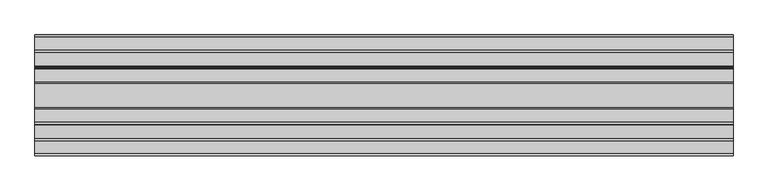
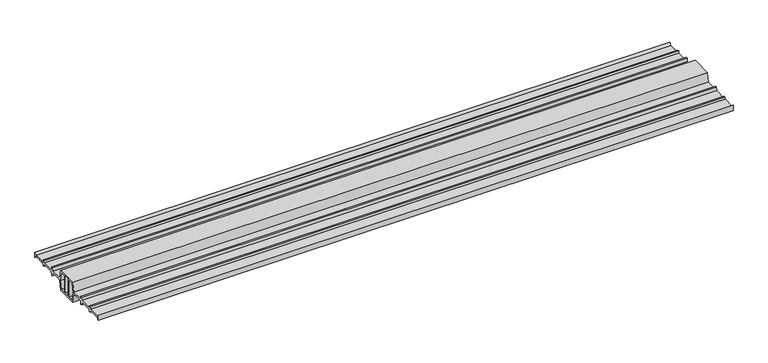
"""IFC4 building model written with IfcOpenShell, lengths in millimetres: proxy geometry, TN_ПВХ_ТПО_Гидрошпонка ТехноНИКОЛЬ : ПВХ Гидрошпонка ТехноНИКОЛЬ IM-260/50."""

import ifcopenshell
import ifcopenshell.guid

model = None  # the IFC model being written
_history = None  # IfcOwnerHistory: only IFC2X3 demands one
_inside = {}  # id of a spatial element -> (the spatial element, [elements in it])
_under = {}  # id of a project, library or spatial element -> (it, [spatial elements below it])
_declared = {}  # id of a project -> (the project, [libraries it declares])
_typed = {}  # id of a type object -> (the type object, [elements of that type])
_made_of = {}  # id of a material, layer set ... -> (it, [elements and type objects made of it])


def new_model(schema):
    """Start an empty IFC model of exactly this schema.

    Asked for "IFC4X3", IfcOpenShell would pick the latest addendum, in which some entities
    have other attributes; the version numbers below select the first issue.
    IFC2X3 requires an IfcOwnerHistory on every rooted entity: one is made here for all.
    """
    global model, _history
    if schema == "IFC4X3":
        model = ifcopenshell.file(schema_version=(4, 3, 0, 0))
    else:
        model = ifcopenshell.file(schema=schema)
    _inside.clear()
    _under.clear()
    _declared.clear()
    _typed.clear()
    _made_of.clear()
    _history = None
    if model.schema == "IFC2X3":
        org = make("IfcOrganization", Name="unknown")
        user = make(
            "IfcPersonAndOrganization",
            ThePerson=make("IfcPerson", FamilyName="unknown"),
            TheOrganization=org,
        )
        app = make(
            "IfcApplication",
            ApplicationDeveloper=org,
            Version="unknown",
            ApplicationFullName="unknown",
            ApplicationIdentifier="unknown",
        )
        _history = make(
            "IfcOwnerHistory",
            OwningUser=user,
            OwningApplication=app,
            ChangeAction="ADDED",
            CreationDate=0,
        )
    return model


def make(cls, **values):
    """One entity of the class cls with the attributes given. An attribute that is None is left unset."""
    return model.create_entity(
        cls, **{name: value for name, value in values.items() if value is not None}
    )


def rooted(cls, **values):
    """An entity with a GlobalId (a new one), such as an element, a storey or a relation."""
    return make(cls, GlobalId=ifcopenshell.guid.new(), OwnerHistory=_history, **values)


def si_unit(unit_type, name, prefix=None):
    """IfcSIUnit, for example si_unit("LENGTHUNIT", "METRE", prefix="MILLI")."""
    return make("IfcSIUnit", UnitType=unit_type, Prefix=prefix, Name=name)


def assignment(units):
    """IfcUnitAssignment: the units of a project."""
    return None if units is None else make("IfcUnitAssignment", Units=units)


def point(xyz):
    """IfcCartesianPoint."""
    return None if xyz is None else make("IfcCartesianPoint", Coordinates=xyz)


def direction(xyz):
    """IfcDirection."""
    return None if xyz is None else make("IfcDirection", DirectionRatios=xyz)


def frame(location, z_axis=None, x_axis=None):
    """IfcAxis2Placement3D, a coordinate frame: its origin and axes. An axis left out is left unset."""
    return make(
        "IfcAxis2Placement3D",
        Location=point(location),
        Axis=direction(z_axis),
        RefDirection=direction(x_axis),
    )


def origin():
    """The frame at (0, 0, 0) with its axes left unset."""
    return frame((0.0, 0.0, 0.0))


def place(relative_to, where):
    """IfcLocalPlacement: puts the frame where relative to a parent placement (None: the world)."""
    return make(
        "IfcLocalPlacement", PlacementRelTo=relative_to, RelativePlacement=where
    )


def context(
    kind, dimensions, precision=None, world=None, true_north=None, identifier=None
):
    """IfcGeometricRepresentationContext, for example the 3D "Model" context."""
    return make(
        "IfcGeometricRepresentationContext",
        ContextIdentifier=identifier,
        ContextType=kind,
        CoordinateSpaceDimension=dimensions,
        Precision=precision,
        WorldCoordinateSystem=world,
        TrueNorth=true_north,
    )


def project(units=None, contexts=None):
    """IfcProject with its units and contexts."""
    return rooted(
        "IfcProject",
        Name="project",
        RepresentationContexts=contexts,
        UnitsInContext=assignment(units),
    )


def spatial(cls, under=None, at=None, **own):
    """A site, building, storey or space (cls), placed at a placement, below another one or the project."""
    s = rooted(cls, ObjectPlacement=at, **own)
    if under is not None:
        _under.setdefault(under.id(), (under, []))[1].append(s)
    return s


def polyline(points):
    """IfcPolyline through the points."""
    return make("IfcPolyline", Points=[point(p) for p in points])


def outline(outer, holes=None, kind="AREA"):
    """IfcArbitraryClosedProfileDef: a profile drawn as a closed curve; with holes, ...WithVoids."""
    if holes is None:
        return make("IfcArbitraryClosedProfileDef", ProfileType=kind, OuterCurve=outer)
    return make(
        "IfcArbitraryProfileDefWithVoids",
        ProfileType=kind,
        OuterCurve=outer,
        InnerCurves=holes,
    )


def extrude(swept, where, along, depth):
    """IfcExtrudedAreaSolid: the profile swept, set in the frame where, extruded along a direction by depth."""
    return make(
        "IfcExtrudedAreaSolid",
        SweptArea=swept,
        Position=where,
        ExtrudedDirection=direction(along),
        Depth=depth,
    )


def shape(context_of_items, identifier, shape_type, items):
    """IfcShapeRepresentation: the items that make up one representation, for example the "Body"."""
    return make(
        "IfcShapeRepresentation",
        ContextOfItems=context_of_items,
        RepresentationIdentifier=identifier,
        RepresentationType=shape_type,
        Items=items,
    )


def source(mapping_origin, context_of_items, identifier, shape_type, items):
    """IfcRepresentationMap: a shape defined once, which mapped items show again and again."""
    return make(
        "IfcRepresentationMap",
        MappingOrigin=mapping_origin,
        MappedRepresentation=shape(context_of_items, identifier, shape_type, items),
    )


def transform(
    local_origin,
    x_axis=None,
    y_axis=None,
    z_axis=None,
    scale=None,
    scale2=None,
    scale3=None,
    uniform=True,
):
    """IfcCartesianTransformationOperator3D, or its non-uniform kind. x_axis, y_axis, z_axis: its Axis1, 2, 3."""
    if uniform:
        return make(
            "IfcCartesianTransformationOperator3D",
            Axis1=direction(x_axis),
            Axis2=direction(y_axis),
            LocalOrigin=point(local_origin),
            Scale=scale,
            Axis3=direction(z_axis),
        )
    return make(
        "IfcCartesianTransformationOperator3DnonUniform",
        Axis1=direction(x_axis),
        Axis2=direction(y_axis),
        LocalOrigin=point(local_origin),
        Scale=scale,
        Axis3=direction(z_axis),
        Scale2=scale2,
        Scale3=scale3,
    )


def mapped(mapping_source, mapping_target):
    """IfcMappedItem: shows the shape of a source again, moved by a transform."""
    return make(
        "IfcMappedItem", MappingSource=mapping_source, MappingTarget=mapping_target
    )


def made_of(thing, what):
    """Note that an element or type object is made of a material, layer set ...; save() writes the relation."""
    if what is not None:
        _made_of.setdefault(what.id(), (what, []))[1].append(thing)
    return thing


def element(
    cls,
    number,
    at=None,
    inside=None,
    cuts=None,
    type_object=None,
    material=None,
    context=None,
    identifier="Body",
    shape_type=None,
    held_by="IfcProductDefinitionShape",
    body=None,
    shapes=None,
    **own,
):
    """One element of the class cls, such as IfcWall. Its Tag is "e" and its number.

    at: its placement. inside: the storey or other place that contains it. cuts: it is an
    opening in that element (IfcRelVoidsElement). A single representation is given by context,
    identifier, shape_type and body (its items); several are given by shapes. held_by: the class
    of the entity that holds the representations. save() writes the other relations.
    """
    e = rooted(cls, Tag="e%d" % number, ObjectPlacement=at, **own)
    if body is not None:
        shapes = [shape(context, identifier, shape_type, body)]
    if shapes is not None:
        e.Representation = make(held_by, Representations=shapes)
    if inside is not None:
        _inside.setdefault(inside.id(), (inside, []))[1].append(e)
    if cuts is not None:
        rooted(
            "IfcRelVoidsElement", RelatingBuildingElement=cuts, RelatedOpeningElement=e
        )
    if type_object is not None:
        _typed.setdefault(type_object.id(), (type_object, []))[1].append(e)
    return made_of(e, material)


def aggregate(whole, parts):
    """IfcRelAggregates: a whole, such as a stair, and the parts it consists of."""
    return rooted("IfcRelAggregates", RelatingObject=whole, RelatedObjects=parts)


def save(model, path):
    """Write the relations noted so far, then the file.

    IfcRelAggregates (storeys below a building ...), IfcRelContainedInSpatialStructure (elements
    in a storey), IfcRelDefinesByType, IfcRelAssociatesMaterial and IfcRelDeclares: one each for
    every whole, place, type object, material and project.
    """
    for whole, parts in _under.values():
        aggregate(whole, parts)
    for where, things in _inside.values():
        rooted(
            "IfcRelContainedInSpatialStructure",
            RelatedElements=things,
            RelatingStructure=where,
        )
    for kind, things in _typed.values():
        rooted("IfcRelDefinesByType", RelatedObjects=things, RelatingType=kind)
    for what, things in _made_of.values():
        rooted("IfcRelAssociatesMaterial", RelatedObjects=things, RelatingMaterial=what)
    for by, libraries in _declared.values():
        rooted("IfcRelDeclares", RelatingContext=by, RelatedDefinitions=libraries)
    model.write(path)


def specialty_equipment_f74244cd(model_context):
    return source(origin(), model_context, "Body", "SweptSolid", [
        extrude(outline(polyline([(-29.1143568, 0.0), (-56.8860421, 0.0), (-58.1581338, -7.7258715), (-61.8418662, -7.7258715), (-63.1139579, 0.0), (-92.2655559, 0.0), (-93.1337968, -4.9240388), (-96.8662032, -4.9240388), (-97.7344441, 0.0), (-125.0007615, 0.0), (-130.0, -4.9992385), (-130.0, 8.0355304), (-125.0007615, 3.0362919), (-97.7344441, 3.5995026), (-96.8662032, 8.8726426), (-93.1337968, 8.8726426), (-92.2823364, 3.6946695), (-63.1111586, 4.2911296), (-61.8418662, 12.0), (-58.1581338, 12.0), (-56.9066733, 4.3994293), (-28.9016162, 4.5391581), (-25.0, 26.6663231), (25.0, 26.6663231), (28.9016162, 4.5391581), (56.9066733, 4.3994293), (58.1581338, 12.0), (61.8418662, 12.0), (63.1111586, 4.2911296), (92.2823364, 3.6946695), (93.1337968, 8.8726426), (96.8662032, 8.8726426), (97.7344441, 3.5995026), (125.0007615, 3.0362919), (130.0, 8.0355304), (130.0, -4.9992385), (125.0007615, 0.0), (97.7344441, 0.0), (96.8662032, -4.9240388), (93.1337968, -4.9240388), (92.2655559, 0.0), (63.1139579, 0.0), (61.8418662, -7.7258715), (58.1581338, -7.7258715), (56.8860421, 0.0), (29.1143568, 0.0), (25.0, -23.3336769), (-25.0, -23.3336769), (-29.1143568, 0.0)]), holes=[polyline([(24.3310415, 1.6663231), (20.8045018, 21.6663231), (10.0, 21.6663231), (10.0, -18.3336769), (20.8045018, -18.3336769), (24.3310415, 1.6663231)]), polyline([(-5.0, -18.3336769), (5.0, -18.3336769), (5.0, 24.6663231), (-5.0, 24.6663231), (-5.0, -18.3336769)]), polyline([(-24.3310415, 1.6663231), (-20.8045018, -18.3336769), (-10.0, -18.3336769), (-10.0, 21.6663231), (-20.8045018, 21.6663231), (-24.3310415, 1.6663231)])]), frame((0.0115641, 0.0, 0.0), z_axis=(1.0, 0.0, 0.0), x_axis=(0.0, 1.0, 0.0)), (0.0, 0.0, 1.0), 1500.0),
    ])


if __name__ == "__main__":
    model = new_model("IFC4")
    model_context = context("Model", 3, world=origin())
    ifc_project = project(units=[si_unit("LENGTHUNIT", "METRE", prefix="MILLI")], contexts=[model_context])
    site = spatial("IfcSite", under=ifc_project)
    building = spatial("IfcBuilding", under=site)
    placement = place(None, origin())
    specialty_equipment_shape = specialty_equipment_f74244cd(model_context)
    element("IfcBuildingElementProxy", 1, Name="TN_ПВХ_ТПО_Гидрошпонка ТехноНИКОЛЬ : ПВХ Гидрошпонка ТехноНИКОЛЬ IM-260/50", ObjectType="TN_ПВХ_ТПО_Гидрошпонка ТехноНИКОЛЬ : ПВХ Гидрошпонка ТехноНИКОЛЬ IM-260/50", at=placement, inside=building, context=model_context, shape_type="MappedRepresentation", body=[
        mapped(specialty_equipment_shape, transform((0.0, 0.0, 0.0), x_axis=(1.0, 0.0, 0.0), y_axis=(0.0, 1.0, 0.0), z_axis=(0.0, 0.0, 1.0))),
    ])
    save(model, "model.ifc")

# Revit data of these elements
# Type "TN_ПВХ_ТПО_Гидрошпонка ТехноНИКОЛЬ : ПВХ Гидрошпонка ТехноНИКОЛЬ IM-260/50"
#   Description = "Внутренняя деформационная ПВХ гидрошпонка. Применяется для герметизации деформационных швов при строительстве заглубленных и подземных сооружений. Ширина деформационного узла 50 мм."
#   Type Comments = "п.м."
#   Manufacturer = "ТехноНИКОЛЬ"
#   URL = "https://www.tn.ru/catalogue/dopolnitelnye_element2/gidroizoljacionnaja_shponka_tipa_dv_320_20/"
#   ADSK_Примечание = ""
#   ADSK_Обозначение [instance default] = "ТехноНИКОЛЬ"
#   ADSK_Наименование = "ПВХ Гидрошпонка ТехноНИКОЛЬ IM-260/50, 10м/рул"
#   ADSK_Масса_Текст = ""
#   ADSK_Марка = ""
#   ADSK_Код изделия = "499187"
#   ADSK_Завод-изготовитель [instance default] = "ТехноНИКОЛЬ"
#   ADSK_Единица измерения [instance default] = "п.м."
#   ADSK_Группирование = "Гидрошпонки"
#   ADSK_URL страницы изделия = "https://www.tn.ru/catalogue/dopolnitelnye_element2/gidroizoljacionnaja_shponka_tipa_dv_320_20/"
#   ADSK_URL документации изделия = "https://nav.tn.ru/upload/iblock/67f/Katalog-i-rekomendatsii-po-primeneniyu_Gidroshponki-TEKHNONIKOL.PDF"
#   built-in parameter 1001306 [instance default] = 3.28084 (stored number, unit not read)
#   ADSK_Размер_Длина [instance default] = 1000 mm
#   ADSK_Количество [instance default] = 1
#   ПВХ_ТПО Гидрошпонка ТехноНИКОЛЬ EC-320-4 = no
#   ПВХ Гидрошпонка ТехноНИКОЛЬ IM-260/50 = yes
#   ПВХ Гидрошпонка ТехноНИКОЛЬ IM-240/20 = no
#   ПВХ Гидрошпонка ТехноНИКОЛЬ IC-240-6 = no
#   ПВХ Гидрошпонка ТехноНИКОЛЬ IC-125-2SP = no
#   ПВХ Гидрошпонка ТехноНИКОЛЬ EM-260/50 = no
#   ПВХ Гидрошпонка ТехноНИКОЛЬ EM-260/20 = no
#   ПВХ Гидрошпонка ТехноНИКОЛЬ EC-320-4 = no
#   ПВХ Гидрошпонка ТехноНИКОЛЬ EC-220-3 = no
#   ПВХ_ТПО Гидрошпонка ТехноНИКОЛЬ EC-220-3 = no
#   ПВХ Гидрошпонка ТехноНИКОЛЬ IC-240-2 = no
#   Материал = TN_ПВХ_Черный
#   Default Elevation = 0
# Element 1 (IfcBuildingElementProxy, "TN_ПВХ_ТПО_Гидрошпонка ТехноНИКОЛЬ : ПВХ Гидрошпонка ТехноНИКОЛЬ IM-260/50")
#   built-in parameter 1001306 = 4.92126 (stored number, unit not read)
#   ADSK_Размер_Длина = 1500 mm
#   ADSK_Количество = 1.5
#   Materials on its faces: "TN_ПВХ_Черный"
# Materials
#   "TN_ПВХ_Черный": class "Типовые", colour RGB 48 48 48, transparency 0, Cost = 0
